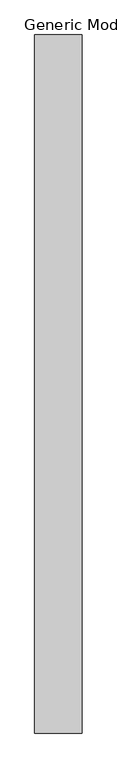
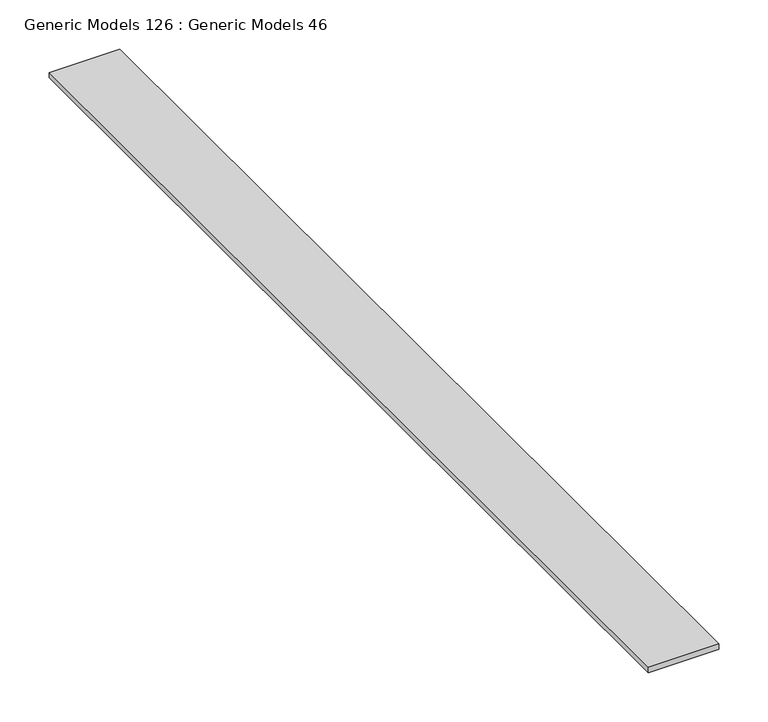
"""IFC4 building model written with IfcOpenShell, lengths in millimetres: proxy geometry, Generic Models 126 : Generic Models 46."""

from ifc_helpers import new_model, si_unit, frame, origin, place, context, project, spatial, polyline, outline, extrude, source, transform, mapped, element, save


def generic_models_126_generic_models_46_0916fb4e(model_context):
    return source(origin(), model_context, "Body", "SweptSolid", [
        extrude(outline(polyline([(48150.8590144, 0.0), (48067.9695022, 0.0), (48067.9695022, 1219.2), (48150.8590144, 1219.2), (48150.8590144, 0.0)])), frame((0.0, 0.0, 999.573933), z_axis=(0.0, 0.0, 1.0), x_axis=(1.0, 0.0, 0.0)), (0.0, 0.0, 1.0), 6.5484375),
    ])


if __name__ == "__main__":
    model = new_model("IFC4")
    model_context = context("Model", 3, world=origin())
    ifc_project = project(units=[si_unit("LENGTHUNIT", "METRE", prefix="MILLI")], contexts=[model_context])
    site = spatial("IfcSite", under=ifc_project)
    building = spatial("IfcBuilding", under=site)
    placement = place(None, origin())
    generic_models_126_generic_models_46_shape = generic_models_126_generic_models_46_0916fb4e(model_context)
    element("IfcBuildingElementProxy", 1, Name="Generic Models 126 : Generic Models 46", ObjectType="Generic Models 126 : Generic Models 46", at=placement, inside=building, context=model_context, shape_type="MappedRepresentation", body=[
        mapped(generic_models_126_generic_models_46_shape, transform((0.0, 0.0, 0.0), x_axis=(1.0, 0.0, 0.0), y_axis=(0.0, 1.0, 0.0), z_axis=(0.0, 0.0, 1.0))),
    ])
    save(model, "model.ifc")

# Revit data of these elements
# Element 1 (IfcBuildingElementProxy, "Generic Models 126 : Generic Models 46")
#   Materials on its faces: "BLOCKING - SIZE AS NEC."
# Materials
#   "BLOCKING - SIZE AS NEC.": class "Wood", colour RGB 234 198 147, transparency 0, Description = "Pinus Echinata", Cost = 0
